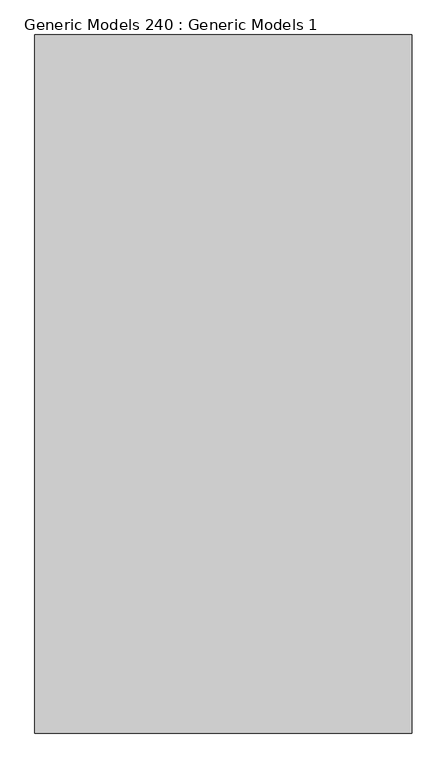
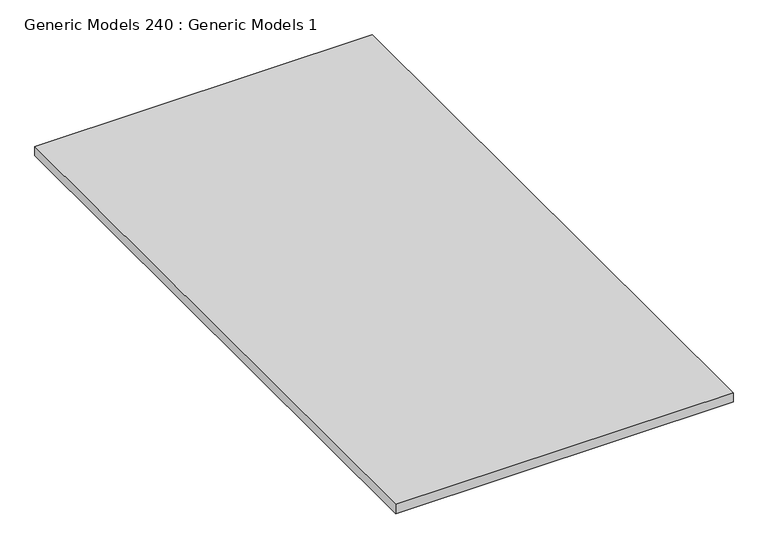
"""IFC4 building model written with IfcOpenShell, lengths in millimetres: proxy geometry, Generic Models 240 : Generic Models 1."""

from ifc_helpers import new_model, si_unit, frame, origin, place, context, project, spatial, polyline, outline, extrude, source, transform, mapped, element, save


def generic_models_240_generic_models_1_611786cf(model_context):
    return source(origin(), model_context, "Body", "SweptSolid", [
        extrude(outline(polyline([(49128.3625, 1219.2), (49128.3625, 0.0), (48469.55, 0.0), (48469.55, 1219.2), (49128.3625, 1219.2)])), frame((0.0, 0.0, 5649.9125), z_axis=(0.0, 0.0, 1.0), x_axis=(1.0, 0.0, 0.0)), (0.0, 0.0, 1.0), 19.05),
    ])


if __name__ == "__main__":
    model = new_model("IFC4")
    model_context = context("Model", 3, world=origin())
    ifc_project = project(units=[si_unit("LENGTHUNIT", "METRE", prefix="MILLI")], contexts=[model_context])
    site = spatial("IfcSite", under=ifc_project)
    building = spatial("IfcBuilding", under=site)
    placement = place(None, origin())
    generic_models_240_generic_models_1_shape = generic_models_240_generic_models_1_611786cf(model_context)
    element("IfcBuildingElementProxy", 1, Name="Generic Models 240 : Generic Models 1", ObjectType="Generic Models 240 : Generic Models 1", at=placement, inside=building, context=model_context, shape_type="MappedRepresentation", body=[
        mapped(generic_models_240_generic_models_1_shape, transform((0.0, 0.0, 0.0), x_axis=(1.0, 0.0, 0.0), y_axis=(0.0, 1.0, 0.0), z_axis=(0.0, 0.0, 1.0))),
    ])
    save(model, "model.ifc")

# Revit data of these elements
# Element 1 (IfcBuildingElementProxy, "Generic Models 240 : Generic Models 1")
#   Materials on its faces: "EXISTING SUBSTRATE"
# Materials
#   "EXISTING SUBSTRATE": class "Unassigned", colour RGB 196 177 123, transparency 0, Cost = 0
